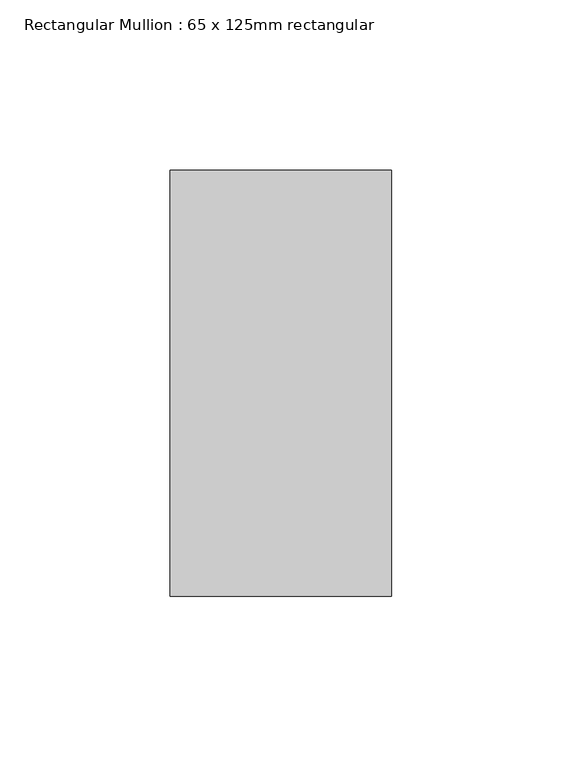
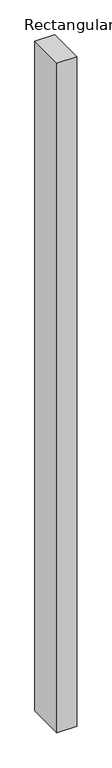
"""IFC4 building model written with IfcOpenShell, lengths in millimetres: member geometry, Rectangular Mullion : 65 x 125mm rectangular."""

from ifc_helpers import new_model, si_unit, frame, origin, place, context, project, spatial, polyline, outline, extrude, source, transform, mapped, element, save


def rectangular_mullion_65_x_125mm_rectangular_64dbaea3(model_context):
    return source(origin(), model_context, "Body", "SweptSolid", [
        extrude(outline(polyline([(0.0, 62.5), (0.0, -62.5), (-65.0, -62.5), (-65.0, 62.5), (0.0, 62.5)])), frame((0.0, 0.0, -2324.4433294), z_axis=(0.0, 0.0, 1.0), x_axis=(1.0, 0.0, 0.0)), (0.0, 0.0, 1.0), 2324.4433294),
    ])


if __name__ == "__main__":
    model = new_model("IFC4")
    model_context = context("Model", 3, world=origin())
    ifc_project = project(units=[si_unit("LENGTHUNIT", "METRE", prefix="MILLI")], contexts=[model_context])
    site = spatial("IfcSite", under=ifc_project)
    building = spatial("IfcBuilding", under=site)
    placement = place(None, origin())
    rectangular_mullion_65_x_125mm_rectangular_shape = rectangular_mullion_65_x_125mm_rectangular_64dbaea3(model_context)
    element("IfcMember", 1, ObjectType="Rectangular Mullion : 65 x 125mm rectangular", at=placement, inside=building, context=model_context, shape_type="MappedRepresentation", body=[
        mapped(rectangular_mullion_65_x_125mm_rectangular_shape, transform((0.0, 0.0, 0.0), x_axis=(1.0, 0.0, 0.0), y_axis=(0.0, 1.0, 0.0), z_axis=(0.0, 0.0, 1.0))),
    ])
    save(model, "model.ifc")

# Revit data of these elements
# Type "Rectangular Mullion : 65 x 125mm rectangular"
#   built-in parameter 1007304 = 0.410105 (stored number, unit not read)
#   built-in parameter 1007301 = 0.106627 (stored number, unit not read)
#   built-in parameter 1007300 = 0.106627 (stored number, unit not read)
# Element 1 (IfcMember, "Rectangular Mullion : 65 x 125mm rectangular")
#   Materials on its faces: "Aluminum"
# Materials
#   "Aluminum": class "Metal", colour RGB 244 245 246, transparency 0, Description = "Aluminum 6061", Cost = 0
